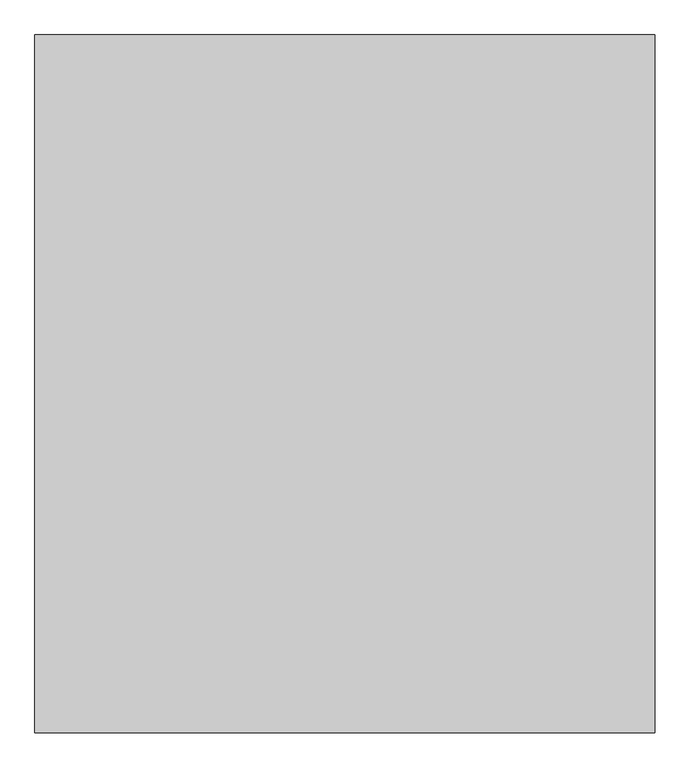
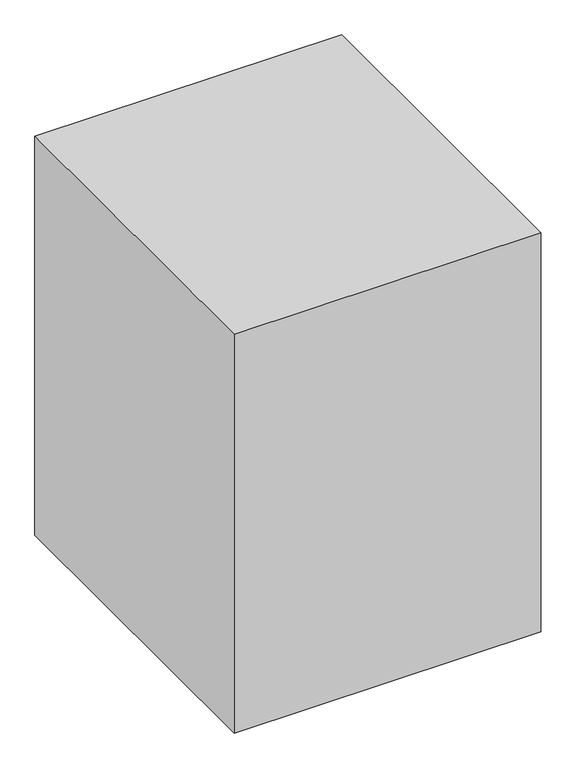
"""IFC4 building model written with IfcOpenShell, lengths in millimetres: proxy geometry, Space Planning Box_hec : Space Planning Box_hec."""

import ifcopenshell
import ifcopenshell.guid

model = None  # the IFC model being written
_history = None  # IfcOwnerHistory: only IFC2X3 demands one
_inside = {}  # id of a spatial element -> (the spatial element, [elements in it])
_under = {}  # id of a project, library or spatial element -> (it, [spatial elements below it])
_declared = {}  # id of a project -> (the project, [libraries it declares])
_typed = {}  # id of a type object -> (the type object, [elements of that type])
_made_of = {}  # id of a material, layer set ... -> (it, [elements and type objects made of it])


def new_model(schema):
    """Start an empty IFC model of exactly this schema.

    Asked for "IFC4X3", IfcOpenShell would pick the latest addendum, in which some entities
    have other attributes; the version numbers below select the first issue.
    IFC2X3 requires an IfcOwnerHistory on every rooted entity: one is made here for all.
    """
    global model, _history
    if schema == "IFC4X3":
        model = ifcopenshell.file(schema_version=(4, 3, 0, 0))
    else:
        model = ifcopenshell.file(schema=schema)
    _inside.clear()
    _under.clear()
    _declared.clear()
    _typed.clear()
    _made_of.clear()
    _history = None
    if model.schema == "IFC2X3":
        org = make("IfcOrganization", Name="unknown")
        user = make(
            "IfcPersonAndOrganization",
            ThePerson=make("IfcPerson", FamilyName="unknown"),
            TheOrganization=org,
        )
        app = make(
            "IfcApplication",
            ApplicationDeveloper=org,
            Version="unknown",
            ApplicationFullName="unknown",
            ApplicationIdentifier="unknown",
        )
        _history = make(
            "IfcOwnerHistory",
            OwningUser=user,
            OwningApplication=app,
            ChangeAction="ADDED",
            CreationDate=0,
        )
    return model


def make(cls, **values):
    """One entity of the class cls with the attributes given. An attribute that is None is left unset."""
    return model.create_entity(
        cls, **{name: value for name, value in values.items() if value is not None}
    )


def rooted(cls, **values):
    """An entity with a GlobalId (a new one), such as an element, a storey or a relation."""
    return make(cls, GlobalId=ifcopenshell.guid.new(), OwnerHistory=_history, **values)


def si_unit(unit_type, name, prefix=None):
    """IfcSIUnit, for example si_unit("LENGTHUNIT", "METRE", prefix="MILLI")."""
    return make("IfcSIUnit", UnitType=unit_type, Prefix=prefix, Name=name)


def assignment(units):
    """IfcUnitAssignment: the units of a project."""
    return None if units is None else make("IfcUnitAssignment", Units=units)


def point(xyz):
    """IfcCartesianPoint."""
    return None if xyz is None else make("IfcCartesianPoint", Coordinates=xyz)


def direction(xyz):
    """IfcDirection."""
    return None if xyz is None else make("IfcDirection", DirectionRatios=xyz)


def frame(location, z_axis=None, x_axis=None):
    """IfcAxis2Placement3D, a coordinate frame: its origin and axes. An axis left out is left unset."""
    return make(
        "IfcAxis2Placement3D",
        Location=point(location),
        Axis=direction(z_axis),
        RefDirection=direction(x_axis),
    )


def origin():
    """The frame at (0, 0, 0) with its axes left unset."""
    return frame((0.0, 0.0, 0.0))


def origin_with_axes():
    """The frame at (0, 0, 0) with the z axis (0, 0, 1) and the x axis (1, 0, 0) written out."""
    return frame((0.0, 0.0, 0.0), z_axis=(0.0, 0.0, 1.0), x_axis=(1.0, 0.0, 0.0))


def place(relative_to, where):
    """IfcLocalPlacement: puts the frame where relative to a parent placement (None: the world)."""
    return make(
        "IfcLocalPlacement", PlacementRelTo=relative_to, RelativePlacement=where
    )


def context(
    kind, dimensions, precision=None, world=None, true_north=None, identifier=None
):
    """IfcGeometricRepresentationContext, for example the 3D "Model" context."""
    return make(
        "IfcGeometricRepresentationContext",
        ContextIdentifier=identifier,
        ContextType=kind,
        CoordinateSpaceDimension=dimensions,
        Precision=precision,
        WorldCoordinateSystem=world,
        TrueNorth=true_north,
    )


def project(units=None, contexts=None):
    """IfcProject with its units and contexts."""
    return rooted(
        "IfcProject",
        Name="project",
        RepresentationContexts=contexts,
        UnitsInContext=assignment(units),
    )


def spatial(cls, under=None, at=None, **own):
    """A site, building, storey or space (cls), placed at a placement, below another one or the project."""
    s = rooted(cls, ObjectPlacement=at, **own)
    if under is not None:
        _under.setdefault(under.id(), (under, []))[1].append(s)
    return s


def polyline(points):
    """IfcPolyline through the points."""
    return make("IfcPolyline", Points=[point(p) for p in points])


def outline(outer, holes=None, kind="AREA"):
    """IfcArbitraryClosedProfileDef: a profile drawn as a closed curve; with holes, ...WithVoids."""
    if holes is None:
        return make("IfcArbitraryClosedProfileDef", ProfileType=kind, OuterCurve=outer)
    return make(
        "IfcArbitraryProfileDefWithVoids",
        ProfileType=kind,
        OuterCurve=outer,
        InnerCurves=holes,
    )


def extrude(swept, where, along, depth):
    """IfcExtrudedAreaSolid: the profile swept, set in the frame where, extruded along a direction by depth."""
    return make(
        "IfcExtrudedAreaSolid",
        SweptArea=swept,
        Position=where,
        ExtrudedDirection=direction(along),
        Depth=depth,
    )


def shape(context_of_items, identifier, shape_type, items):
    """IfcShapeRepresentation: the items that make up one representation, for example the "Body"."""
    return make(
        "IfcShapeRepresentation",
        ContextOfItems=context_of_items,
        RepresentationIdentifier=identifier,
        RepresentationType=shape_type,
        Items=items,
    )


def source(mapping_origin, context_of_items, identifier, shape_type, items):
    """IfcRepresentationMap: a shape defined once, which mapped items show again and again."""
    return make(
        "IfcRepresentationMap",
        MappingOrigin=mapping_origin,
        MappedRepresentation=shape(context_of_items, identifier, shape_type, items),
    )


def transform(
    local_origin,
    x_axis=None,
    y_axis=None,
    z_axis=None,
    scale=None,
    scale2=None,
    scale3=None,
    uniform=True,
):
    """IfcCartesianTransformationOperator3D, or its non-uniform kind. x_axis, y_axis, z_axis: its Axis1, 2, 3."""
    if uniform:
        return make(
            "IfcCartesianTransformationOperator3D",
            Axis1=direction(x_axis),
            Axis2=direction(y_axis),
            LocalOrigin=point(local_origin),
            Scale=scale,
            Axis3=direction(z_axis),
        )
    return make(
        "IfcCartesianTransformationOperator3DnonUniform",
        Axis1=direction(x_axis),
        Axis2=direction(y_axis),
        LocalOrigin=point(local_origin),
        Scale=scale,
        Axis3=direction(z_axis),
        Scale2=scale2,
        Scale3=scale3,
    )


def mapped(mapping_source, mapping_target):
    """IfcMappedItem: shows the shape of a source again, moved by a transform."""
    return make(
        "IfcMappedItem", MappingSource=mapping_source, MappingTarget=mapping_target
    )


def made_of(thing, what):
    """Note that an element or type object is made of a material, layer set ...; save() writes the relation."""
    if what is not None:
        _made_of.setdefault(what.id(), (what, []))[1].append(thing)
    return thing


def element(
    cls,
    number,
    at=None,
    inside=None,
    cuts=None,
    type_object=None,
    material=None,
    context=None,
    identifier="Body",
    shape_type=None,
    held_by="IfcProductDefinitionShape",
    body=None,
    shapes=None,
    **own,
):
    """One element of the class cls, such as IfcWall. Its Tag is "e" and its number.

    at: its placement. inside: the storey or other place that contains it. cuts: it is an
    opening in that element (IfcRelVoidsElement). A single representation is given by context,
    identifier, shape_type and body (its items); several are given by shapes. held_by: the class
    of the entity that holds the representations. save() writes the other relations.
    """
    e = rooted(cls, Tag="e%d" % number, ObjectPlacement=at, **own)
    if body is not None:
        shapes = [shape(context, identifier, shape_type, body)]
    if shapes is not None:
        e.Representation = make(held_by, Representations=shapes)
    if inside is not None:
        _inside.setdefault(inside.id(), (inside, []))[1].append(e)
    if cuts is not None:
        rooted(
            "IfcRelVoidsElement", RelatingBuildingElement=cuts, RelatedOpeningElement=e
        )
    if type_object is not None:
        _typed.setdefault(type_object.id(), (type_object, []))[1].append(e)
    return made_of(e, material)


def aggregate(whole, parts):
    """IfcRelAggregates: a whole, such as a stair, and the parts it consists of."""
    return rooted("IfcRelAggregates", RelatingObject=whole, RelatedObjects=parts)


def save(model, path):
    """Write the relations noted so far, then the file.

    IfcRelAggregates (storeys below a building ...), IfcRelContainedInSpatialStructure (elements
    in a storey), IfcRelDefinesByType, IfcRelAssociatesMaterial and IfcRelDeclares: one each for
    every whole, place, type object, material and project.
    """
    for whole, parts in _under.values():
        aggregate(whole, parts)
    for where, things in _inside.values():
        rooted(
            "IfcRelContainedInSpatialStructure",
            RelatedElements=things,
            RelatingStructure=where,
        )
    for kind, things in _typed.values():
        rooted("IfcRelDefinesByType", RelatedObjects=things, RelatingType=kind)
    for what, things in _made_of.values():
        rooted("IfcRelAssociatesMaterial", RelatedObjects=things, RelatingMaterial=what)
    for by, libraries in _declared.values():
        rooted("IfcRelDeclares", RelatingContext=by, RelatedDefinitions=libraries)
    model.write(path)


def generic_models_971c0b89(model_context):
    return source(origin(), model_context, "Body", "SweptSolid", [
        extrude(outline(polyline([(2000.0, 2250.0), (2000.0, -2250.0), (-2000.0, -2250.0), (-2000.0, 2250.0), (2000.0, 2250.0)])), origin_with_axes(), (0.0, 0.0, 1.0), 5500.0),
    ])


if __name__ == "__main__":
    model = new_model("IFC4")
    model_context = context("Model", 3, world=origin())
    ifc_project = project(units=[si_unit("LENGTHUNIT", "METRE", prefix="MILLI")], contexts=[model_context])
    site = spatial("IfcSite", under=ifc_project)
    building = spatial("IfcBuilding", under=site)
    placement = place(None, origin())
    generic_models_shape = generic_models_971c0b89(model_context)
    element("IfcBuildingElementProxy", 1, Name="Space Planning Box_hec : Space Planning Box_hec", ObjectType="Space Planning Box_hec : Space Planning Box_hec", at=placement, inside=building, context=model_context, shape_type="MappedRepresentation", body=[
        mapped(generic_models_shape, transform((0.0, 0.0, 0.0), x_axis=(1.0, 0.0, 0.0), y_axis=(0.0, 1.0, 0.0), z_axis=(0.0, 0.0, 1.0))),
    ])
    save(model, "model.ifc")

# Revit data of these elements
# Type "Space Planning Box_hec : Space Planning Box_hec"
#   Type Comments = "..."
#   Room Name [instance default] = "?"
#   Interior Finish [instance default] = ""
#   Exterior Finish [instance default] = ""
#   Department [instance default] = ""
#   Assembly Code = "..."
#   ceiling height [instance default] = 0
#   Width [instance default] = 1524 mm
#   Program Area [instance default] = 0.00 m²
#   Length [instance default] = 1524 mm
#   Height [instance default] = 1524 mm
#   Area [instance default] = 2.32258 m²
#   Fill Color [instance default] = Cyan
#   Default Elevation = 0
# Element 1 (IfcBuildingElementProxy, "Space Planning Box_hec : Space Planning Box_hec")
#   Room Name = "Toilet (M)"
#   Exterior Finish = "N/A..N/A,,EW2..N/A..N/A"
#   Department = "AR"
#   Width = 4000 mm
#   Program Area = 18.00 m²
#   Length = 4500 mm
#   Height = 5500 mm
#   Area = 18.00 m²
#   Materials on its faces: "Cyan"
# Materials
#   "Cyan": class "Generic", colour RGB 0 255 255, transparency 0.2, Cost = 0
